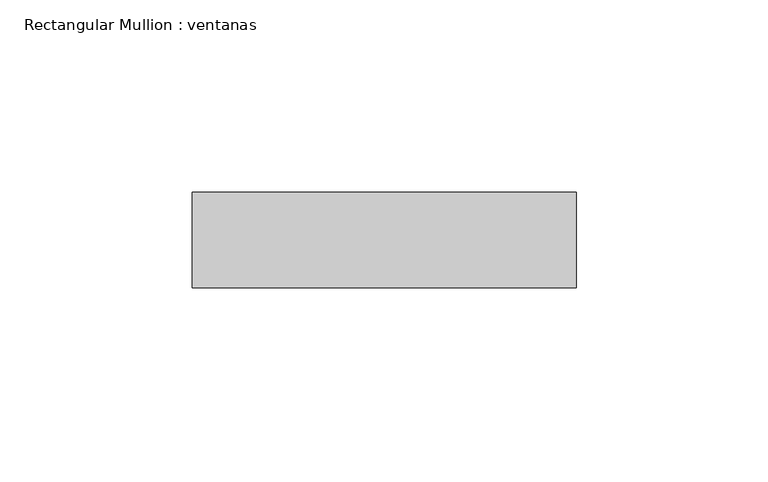
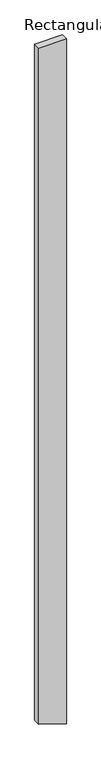
"""IFC4 building model written with IfcOpenShell, lengths in millimetres: member geometry, Rectangular Mullion : ventanas."""

from ifc_helpers import new_model, si_unit, frame, origin, place, context, project, spatial, polyline, outline, extrude, source, transform, mapped, element, save


def rectangular_mullion_ventanas_20222c10(model_context):
    return source(origin(), model_context, "Body", "SweptSolid", [
        extrude(outline(polyline([(0.0, 50.0), (0.0, -50.0), (-2584.3604429, -50.0), (-2612.9562497, 32.6847006), (-2618.9446001, 50.0), (0.0, 50.0)])), frame((0.0, -12.5, 0.0), z_axis=(0.0, 1.0, 0.0), x_axis=(0.0, 0.0, 1.0)), (0.0, 0.0, 1.0), 25.0),
    ])


if __name__ == "__main__":
    model = new_model("IFC4")
    model_context = context("Model", 3, world=origin())
    ifc_project = project(units=[si_unit("LENGTHUNIT", "METRE", prefix="MILLI")], contexts=[model_context])
    site = spatial("IfcSite", under=ifc_project)
    building = spatial("IfcBuilding", under=site)
    placement = place(None, origin())
    rectangular_mullion_ventanas_shape = rectangular_mullion_ventanas_20222c10(model_context)
    element("IfcMember", 1, ObjectType="Rectangular Mullion : ventanas", at=placement, inside=building, context=model_context, shape_type="MappedRepresentation", body=[
        mapped(rectangular_mullion_ventanas_shape, transform((0.0, 0.0, 0.0), x_axis=(1.0, 0.0, 0.0), y_axis=(0.0, 1.0, 0.0), z_axis=(0.0, 0.0, 1.0))),
    ])
    save(model, "model.ifc")

# Revit data of these elements
# Type "Rectangular Mullion : ventanas"
#   built-in parameter 1007304 = 0.082021 (stored number, unit not read)
#   built-in parameter 1007301 = 0.164042 (stored number, unit not read)
#   built-in parameter 1007300 = 0.164042 (stored number, unit not read)
# Element 1 (IfcMember, "Rectangular Mullion : ventanas")
#   Materials on its faces: "Metal Deck"
# Materials
#   "Metal Deck": class "Metal", colour RGB 84 83 81, transparency 0, Description = "Steel, mill finish", Cost = 0
